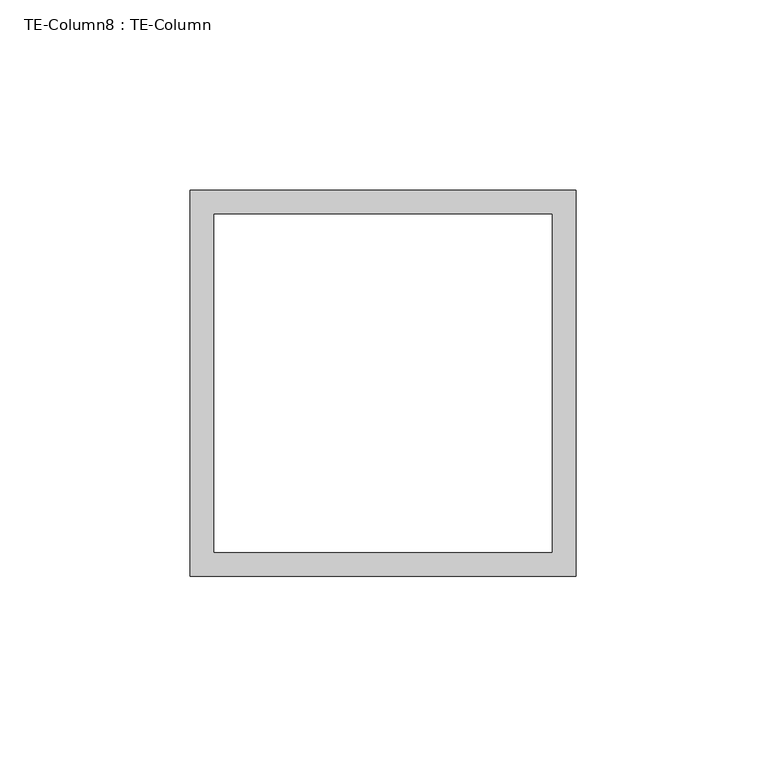
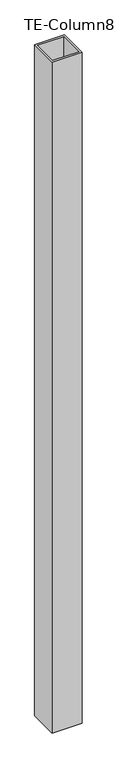
"""IFC4 building model written with IfcOpenShell, lengths in millimetres: proxy geometry, TE-Column8 : TE-Column."""

import ifcopenshell
import ifcopenshell.guid

model = None  # the IFC model being written
_history = None  # IfcOwnerHistory: only IFC2X3 demands one
_inside = {}  # id of a spatial element -> (the spatial element, [elements in it])
_under = {}  # id of a project, library or spatial element -> (it, [spatial elements below it])
_declared = {}  # id of a project -> (the project, [libraries it declares])
_typed = {}  # id of a type object -> (the type object, [elements of that type])
_made_of = {}  # id of a material, layer set ... -> (it, [elements and type objects made of it])


def new_model(schema):
    """Start an empty IFC model of exactly this schema.

    Asked for "IFC4X3", IfcOpenShell would pick the latest addendum, in which some entities
    have other attributes; the version numbers below select the first issue.
    IFC2X3 requires an IfcOwnerHistory on every rooted entity: one is made here for all.
    """
    global model, _history
    if schema == "IFC4X3":
        model = ifcopenshell.file(schema_version=(4, 3, 0, 0))
    else:
        model = ifcopenshell.file(schema=schema)
    _inside.clear()
    _under.clear()
    _declared.clear()
    _typed.clear()
    _made_of.clear()
    _history = None
    if model.schema == "IFC2X3":
        org = make("IfcOrganization", Name="unknown")
        user = make(
            "IfcPersonAndOrganization",
            ThePerson=make("IfcPerson", FamilyName="unknown"),
            TheOrganization=org,
        )
        app = make(
            "IfcApplication",
            ApplicationDeveloper=org,
            Version="unknown",
            ApplicationFullName="unknown",
            ApplicationIdentifier="unknown",
        )
        _history = make(
            "IfcOwnerHistory",
            OwningUser=user,
            OwningApplication=app,
            ChangeAction="ADDED",
            CreationDate=0,
        )
    return model


def make(cls, **values):
    """One entity of the class cls with the attributes given. An attribute that is None is left unset."""
    return model.create_entity(
        cls, **{name: value for name, value in values.items() if value is not None}
    )


def rooted(cls, **values):
    """An entity with a GlobalId (a new one), such as an element, a storey or a relation."""
    return make(cls, GlobalId=ifcopenshell.guid.new(), OwnerHistory=_history, **values)


def si_unit(unit_type, name, prefix=None):
    """IfcSIUnit, for example si_unit("LENGTHUNIT", "METRE", prefix="MILLI")."""
    return make("IfcSIUnit", UnitType=unit_type, Prefix=prefix, Name=name)


def assignment(units):
    """IfcUnitAssignment: the units of a project."""
    return None if units is None else make("IfcUnitAssignment", Units=units)


def point(xyz):
    """IfcCartesianPoint."""
    return None if xyz is None else make("IfcCartesianPoint", Coordinates=xyz)


def direction(xyz):
    """IfcDirection."""
    return None if xyz is None else make("IfcDirection", DirectionRatios=xyz)


def frame(location, z_axis=None, x_axis=None):
    """IfcAxis2Placement3D, a coordinate frame: its origin and axes. An axis left out is left unset."""
    return make(
        "IfcAxis2Placement3D",
        Location=point(location),
        Axis=direction(z_axis),
        RefDirection=direction(x_axis),
    )


def origin():
    """The frame at (0, 0, 0) with its axes left unset."""
    return frame((0.0, 0.0, 0.0))


def place(relative_to, where):
    """IfcLocalPlacement: puts the frame where relative to a parent placement (None: the world)."""
    return make(
        "IfcLocalPlacement", PlacementRelTo=relative_to, RelativePlacement=where
    )


def context(
    kind, dimensions, precision=None, world=None, true_north=None, identifier=None
):
    """IfcGeometricRepresentationContext, for example the 3D "Model" context."""
    return make(
        "IfcGeometricRepresentationContext",
        ContextIdentifier=identifier,
        ContextType=kind,
        CoordinateSpaceDimension=dimensions,
        Precision=precision,
        WorldCoordinateSystem=world,
        TrueNorth=true_north,
    )


def project(units=None, contexts=None):
    """IfcProject with its units and contexts."""
    return rooted(
        "IfcProject",
        Name="project",
        RepresentationContexts=contexts,
        UnitsInContext=assignment(units),
    )


def spatial(cls, under=None, at=None, **own):
    """A site, building, storey or space (cls), placed at a placement, below another one or the project."""
    s = rooted(cls, ObjectPlacement=at, **own)
    if under is not None:
        _under.setdefault(under.id(), (under, []))[1].append(s)
    return s


def polyline(points):
    """IfcPolyline through the points."""
    return make("IfcPolyline", Points=[point(p) for p in points])


def outline(outer, holes=None, kind="AREA"):
    """IfcArbitraryClosedProfileDef: a profile drawn as a closed curve; with holes, ...WithVoids."""
    if holes is None:
        return make("IfcArbitraryClosedProfileDef", ProfileType=kind, OuterCurve=outer)
    return make(
        "IfcArbitraryProfileDefWithVoids",
        ProfileType=kind,
        OuterCurve=outer,
        InnerCurves=holes,
    )


def extrude(swept, where, along, depth):
    """IfcExtrudedAreaSolid: the profile swept, set in the frame where, extruded along a direction by depth."""
    return make(
        "IfcExtrudedAreaSolid",
        SweptArea=swept,
        Position=where,
        ExtrudedDirection=direction(along),
        Depth=depth,
    )


def shape(context_of_items, identifier, shape_type, items):
    """IfcShapeRepresentation: the items that make up one representation, for example the "Body"."""
    return make(
        "IfcShapeRepresentation",
        ContextOfItems=context_of_items,
        RepresentationIdentifier=identifier,
        RepresentationType=shape_type,
        Items=items,
    )


def source(mapping_origin, context_of_items, identifier, shape_type, items):
    """IfcRepresentationMap: a shape defined once, which mapped items show again and again."""
    return make(
        "IfcRepresentationMap",
        MappingOrigin=mapping_origin,
        MappedRepresentation=shape(context_of_items, identifier, shape_type, items),
    )


def transform(
    local_origin,
    x_axis=None,
    y_axis=None,
    z_axis=None,
    scale=None,
    scale2=None,
    scale3=None,
    uniform=True,
):
    """IfcCartesianTransformationOperator3D, or its non-uniform kind. x_axis, y_axis, z_axis: its Axis1, 2, 3."""
    if uniform:
        return make(
            "IfcCartesianTransformationOperator3D",
            Axis1=direction(x_axis),
            Axis2=direction(y_axis),
            LocalOrigin=point(local_origin),
            Scale=scale,
            Axis3=direction(z_axis),
        )
    return make(
        "IfcCartesianTransformationOperator3DnonUniform",
        Axis1=direction(x_axis),
        Axis2=direction(y_axis),
        LocalOrigin=point(local_origin),
        Scale=scale,
        Axis3=direction(z_axis),
        Scale2=scale2,
        Scale3=scale3,
    )


def mapped(mapping_source, mapping_target):
    """IfcMappedItem: shows the shape of a source again, moved by a transform."""
    return make(
        "IfcMappedItem", MappingSource=mapping_source, MappingTarget=mapping_target
    )


def made_of(thing, what):
    """Note that an element or type object is made of a material, layer set ...; save() writes the relation."""
    if what is not None:
        _made_of.setdefault(what.id(), (what, []))[1].append(thing)
    return thing


def element(
    cls,
    number,
    at=None,
    inside=None,
    cuts=None,
    type_object=None,
    material=None,
    context=None,
    identifier="Body",
    shape_type=None,
    held_by="IfcProductDefinitionShape",
    body=None,
    shapes=None,
    **own,
):
    """One element of the class cls, such as IfcWall. Its Tag is "e" and its number.

    at: its placement. inside: the storey or other place that contains it. cuts: it is an
    opening in that element (IfcRelVoidsElement). A single representation is given by context,
    identifier, shape_type and body (its items); several are given by shapes. held_by: the class
    of the entity that holds the representations. save() writes the other relations.
    """
    e = rooted(cls, Tag="e%d" % number, ObjectPlacement=at, **own)
    if body is not None:
        shapes = [shape(context, identifier, shape_type, body)]
    if shapes is not None:
        e.Representation = make(held_by, Representations=shapes)
    if inside is not None:
        _inside.setdefault(inside.id(), (inside, []))[1].append(e)
    if cuts is not None:
        rooted(
            "IfcRelVoidsElement", RelatingBuildingElement=cuts, RelatedOpeningElement=e
        )
    if type_object is not None:
        _typed.setdefault(type_object.id(), (type_object, []))[1].append(e)
    return made_of(e, material)


def aggregate(whole, parts):
    """IfcRelAggregates: a whole, such as a stair, and the parts it consists of."""
    return rooted("IfcRelAggregates", RelatingObject=whole, RelatedObjects=parts)


def save(model, path):
    """Write the relations noted so far, then the file.

    IfcRelAggregates (storeys below a building ...), IfcRelContainedInSpatialStructure (elements
    in a storey), IfcRelDefinesByType, IfcRelAssociatesMaterial and IfcRelDeclares: one each for
    every whole, place, type object, material and project.
    """
    for whole, parts in _under.values():
        aggregate(whole, parts)
    for where, things in _inside.values():
        rooted(
            "IfcRelContainedInSpatialStructure",
            RelatedElements=things,
            RelatingStructure=where,
        )
    for kind, things in _typed.values():
        rooted("IfcRelDefinesByType", RelatedObjects=things, RelatingType=kind)
    for what, things in _made_of.values():
        rooted("IfcRelAssociatesMaterial", RelatedObjects=things, RelatingMaterial=what)
    for by, libraries in _declared.values():
        rooted("IfcRelDeclares", RelatingContext=by, RelatedDefinitions=libraries)
    model.write(path)


def te_column8_te_column_a4862150(model_context):
    return source(origin(), model_context, "Body", "SweptSolid", [
        extrude(outline(polyline([(587365.8934739, -536315.9913841), (587467.4934739, -536315.9913841), (587467.4934739, -536417.5913841), (587365.8934739, -536417.5913841), (587365.8934739, -536315.9913841)]), holes=[polyline([(587372.2434739, -536411.2413841), (587461.1434739, -536411.2413841), (587461.1434739, -536322.3413841), (587372.2434739, -536322.3413841), (587372.2434739, -536411.2413841)])]), frame((0.0, 0.0, 28.575), z_axis=(0.0, 0.0, 1.0), x_axis=(1.0, 0.0, 0.0)), (0.0, 0.0, 1.0), 2406.65),
    ])


if __name__ == "__main__":
    model = new_model("IFC4")
    model_context = context("Model", 3, world=origin())
    ifc_project = project(units=[si_unit("LENGTHUNIT", "METRE", prefix="MILLI")], contexts=[model_context])
    site = spatial("IfcSite", under=ifc_project)
    building = spatial("IfcBuilding", under=site)
    placement = place(None, origin())
    te_column8_te_column_shape = te_column8_te_column_a4862150(model_context)
    element("IfcBuildingElementProxy", 1, Name="TE-Column8 : TE-Column", ObjectType="TE-Column8 : TE-Column", at=placement, inside=building, context=model_context, shape_type="MappedRepresentation", body=[
        mapped(te_column8_te_column_shape, transform((0.0, 0.0, 0.0), x_axis=(1.0, 0.0, 0.0), y_axis=(0.0, 1.0, 0.0), z_axis=(0.0, 0.0, 1.0))),
    ])
    save(model, "model.ifc")

# Revit data of these elements
# Element 1 (IfcBuildingElementProxy, "TE-Column8 : TE-Column")
#   Materials on its faces: "4\"X4\" GALV. HSS TUBING"
# Materials
#   "4\"X4\" GALV. HSS TUBING": class "Generic", colour RGB 211 211 207, transparency 0, Cost = 0
